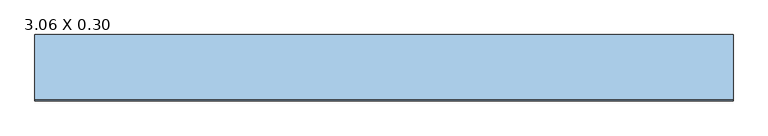
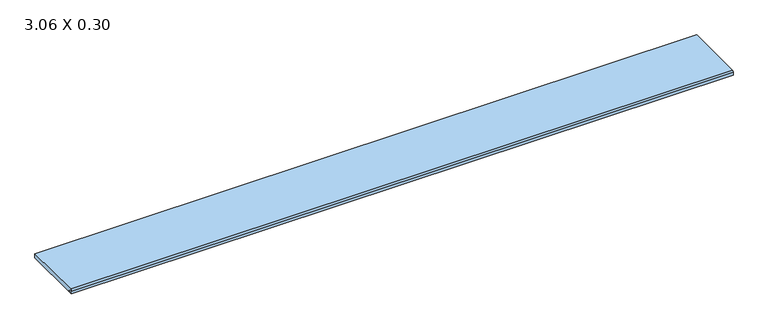
"""IFC4 building model written with IfcOpenShell, lengths in millimetres: window geometry, .CC_ND 300_PEDRA_PEITORIL RETO : 3.06 X 0.30."""

import ifcopenshell
import ifcopenshell.guid

model = None  # the IFC model being written
_history = None  # IfcOwnerHistory: only IFC2X3 demands one
_inside = {}  # id of a spatial element -> (the spatial element, [elements in it])
_under = {}  # id of a project, library or spatial element -> (it, [spatial elements below it])
_declared = {}  # id of a project -> (the project, [libraries it declares])
_typed = {}  # id of a type object -> (the type object, [elements of that type])
_made_of = {}  # id of a material, layer set ... -> (it, [elements and type objects made of it])


def new_model(schema):
    """Start an empty IFC model of exactly this schema.

    Asked for "IFC4X3", IfcOpenShell would pick the latest addendum, in which some entities
    have other attributes; the version numbers below select the first issue.
    IFC2X3 requires an IfcOwnerHistory on every rooted entity: one is made here for all.
    """
    global model, _history
    if schema == "IFC4X3":
        model = ifcopenshell.file(schema_version=(4, 3, 0, 0))
    else:
        model = ifcopenshell.file(schema=schema)
    _inside.clear()
    _under.clear()
    _declared.clear()
    _typed.clear()
    _made_of.clear()
    _history = None
    if model.schema == "IFC2X3":
        org = make("IfcOrganization", Name="unknown")
        user = make(
            "IfcPersonAndOrganization",
            ThePerson=make("IfcPerson", FamilyName="unknown"),
            TheOrganization=org,
        )
        app = make(
            "IfcApplication",
            ApplicationDeveloper=org,
            Version="unknown",
            ApplicationFullName="unknown",
            ApplicationIdentifier="unknown",
        )
        _history = make(
            "IfcOwnerHistory",
            OwningUser=user,
            OwningApplication=app,
            ChangeAction="ADDED",
            CreationDate=0,
        )
    return model


def make(cls, **values):
    """One entity of the class cls with the attributes given. An attribute that is None is left unset."""
    return model.create_entity(
        cls, **{name: value for name, value in values.items() if value is not None}
    )


def rooted(cls, **values):
    """An entity with a GlobalId (a new one), such as an element, a storey or a relation."""
    return make(cls, GlobalId=ifcopenshell.guid.new(), OwnerHistory=_history, **values)


def si_unit(unit_type, name, prefix=None):
    """IfcSIUnit, for example si_unit("LENGTHUNIT", "METRE", prefix="MILLI")."""
    return make("IfcSIUnit", UnitType=unit_type, Prefix=prefix, Name=name)


def assignment(units):
    """IfcUnitAssignment: the units of a project."""
    return None if units is None else make("IfcUnitAssignment", Units=units)


def point(xyz):
    """IfcCartesianPoint."""
    return None if xyz is None else make("IfcCartesianPoint", Coordinates=xyz)


def direction(xyz):
    """IfcDirection."""
    return None if xyz is None else make("IfcDirection", DirectionRatios=xyz)


def frame(location, z_axis=None, x_axis=None):
    """IfcAxis2Placement3D, a coordinate frame: its origin and axes. An axis left out is left unset."""
    return make(
        "IfcAxis2Placement3D",
        Location=point(location),
        Axis=direction(z_axis),
        RefDirection=direction(x_axis),
    )


def frame_2d(location, x_axis=None):
    """IfcAxis2Placement2D, a coordinate frame in the plane: its origin and x axis."""
    return make(
        "IfcAxis2Placement2D", Location=point(location), RefDirection=direction(x_axis)
    )


def origin():
    """The frame at (0, 0, 0) with its axes left unset."""
    return frame((0.0, 0.0, 0.0))


def place(relative_to, where):
    """IfcLocalPlacement: puts the frame where relative to a parent placement (None: the world)."""
    return make(
        "IfcLocalPlacement", PlacementRelTo=relative_to, RelativePlacement=where
    )


def context(
    kind, dimensions, precision=None, world=None, true_north=None, identifier=None
):
    """IfcGeometricRepresentationContext, for example the 3D "Model" context."""
    return make(
        "IfcGeometricRepresentationContext",
        ContextIdentifier=identifier,
        ContextType=kind,
        CoordinateSpaceDimension=dimensions,
        Precision=precision,
        WorldCoordinateSystem=world,
        TrueNorth=true_north,
    )


def project(units=None, contexts=None):
    """IfcProject with its units and contexts."""
    return rooted(
        "IfcProject",
        Name="project",
        RepresentationContexts=contexts,
        UnitsInContext=assignment(units),
    )


def spatial(cls, under=None, at=None, **own):
    """A site, building, storey or space (cls), placed at a placement, below another one or the project."""
    s = rooted(cls, ObjectPlacement=at, **own)
    if under is not None:
        _under.setdefault(under.id(), (under, []))[1].append(s)
    return s


def polyline(points):
    """IfcPolyline through the points."""
    return make("IfcPolyline", Points=[point(p) for p in points])


def circle_curve(where, radius):
    """IfcCircle in the frame where."""
    return make("IfcCircle", Position=where, Radius=radius)


def trimmed(basis, trim1, trim2, sense, master):
    """IfcTrimmedCurve: the piece of a basis curve between two trims."""
    return make(
        "IfcTrimmedCurve",
        BasisCurve=basis,
        Trim1=trim1,
        Trim2=trim2,
        SenseAgreement=sense,
        MasterRepresentation=master,
    )


def segment(curve, same_sense, transition):
    """IfcCompositeCurveSegment."""
    return make(
        "IfcCompositeCurveSegment",
        Transition=transition,
        SameSense=same_sense,
        ParentCurve=curve,
    )


def composite_curve(segments, self_intersect=None):
    """IfcCompositeCurve: segments joined end to end."""
    return make("IfcCompositeCurve", Segments=segments, SelfIntersect=self_intersect)


def outline(outer, holes=None, kind="AREA"):
    """IfcArbitraryClosedProfileDef: a profile drawn as a closed curve; with holes, ...WithVoids."""
    if holes is None:
        return make("IfcArbitraryClosedProfileDef", ProfileType=kind, OuterCurve=outer)
    return make(
        "IfcArbitraryProfileDefWithVoids",
        ProfileType=kind,
        OuterCurve=outer,
        InnerCurves=holes,
    )


def extrude(swept, where, along, depth):
    """IfcExtrudedAreaSolid: the profile swept, set in the frame where, extruded along a direction by depth."""
    return make(
        "IfcExtrudedAreaSolid",
        SweptArea=swept,
        Position=where,
        ExtrudedDirection=direction(along),
        Depth=depth,
    )


def shape(context_of_items, identifier, shape_type, items):
    """IfcShapeRepresentation: the items that make up one representation, for example the "Body"."""
    return make(
        "IfcShapeRepresentation",
        ContextOfItems=context_of_items,
        RepresentationIdentifier=identifier,
        RepresentationType=shape_type,
        Items=items,
    )


def source(mapping_origin, context_of_items, identifier, shape_type, items):
    """IfcRepresentationMap: a shape defined once, which mapped items show again and again."""
    return make(
        "IfcRepresentationMap",
        MappingOrigin=mapping_origin,
        MappedRepresentation=shape(context_of_items, identifier, shape_type, items),
    )


def transform(
    local_origin,
    x_axis=None,
    y_axis=None,
    z_axis=None,
    scale=None,
    scale2=None,
    scale3=None,
    uniform=True,
):
    """IfcCartesianTransformationOperator3D, or its non-uniform kind. x_axis, y_axis, z_axis: its Axis1, 2, 3."""
    if uniform:
        return make(
            "IfcCartesianTransformationOperator3D",
            Axis1=direction(x_axis),
            Axis2=direction(y_axis),
            LocalOrigin=point(local_origin),
            Scale=scale,
            Axis3=direction(z_axis),
        )
    return make(
        "IfcCartesianTransformationOperator3DnonUniform",
        Axis1=direction(x_axis),
        Axis2=direction(y_axis),
        LocalOrigin=point(local_origin),
        Scale=scale,
        Axis3=direction(z_axis),
        Scale2=scale2,
        Scale3=scale3,
    )


def mapped(mapping_source, mapping_target):
    """IfcMappedItem: shows the shape of a source again, moved by a transform."""
    return make(
        "IfcMappedItem", MappingSource=mapping_source, MappingTarget=mapping_target
    )


def made_of(thing, what):
    """Note that an element or type object is made of a material, layer set ...; save() writes the relation."""
    if what is not None:
        _made_of.setdefault(what.id(), (what, []))[1].append(thing)
    return thing


def element(
    cls,
    number,
    at=None,
    inside=None,
    cuts=None,
    type_object=None,
    material=None,
    context=None,
    identifier="Body",
    shape_type=None,
    held_by="IfcProductDefinitionShape",
    body=None,
    shapes=None,
    **own,
):
    """One element of the class cls, such as IfcWall. Its Tag is "e" and its number.

    at: its placement. inside: the storey or other place that contains it. cuts: it is an
    opening in that element (IfcRelVoidsElement). A single representation is given by context,
    identifier, shape_type and body (its items); several are given by shapes. held_by: the class
    of the entity that holds the representations. save() writes the other relations.
    """
    e = rooted(cls, Tag="e%d" % number, ObjectPlacement=at, **own)
    if body is not None:
        shapes = [shape(context, identifier, shape_type, body)]
    if shapes is not None:
        e.Representation = make(held_by, Representations=shapes)
    if inside is not None:
        _inside.setdefault(inside.id(), (inside, []))[1].append(e)
    if cuts is not None:
        rooted(
            "IfcRelVoidsElement", RelatingBuildingElement=cuts, RelatedOpeningElement=e
        )
    if type_object is not None:
        _typed.setdefault(type_object.id(), (type_object, []))[1].append(e)
    return made_of(e, material)


def aggregate(whole, parts):
    """IfcRelAggregates: a whole, such as a stair, and the parts it consists of."""
    return rooted("IfcRelAggregates", RelatingObject=whole, RelatedObjects=parts)


def save(model, path):
    """Write the relations noted so far, then the file.

    IfcRelAggregates (storeys below a building ...), IfcRelContainedInSpatialStructure (elements
    in a storey), IfcRelDefinesByType, IfcRelAssociatesMaterial and IfcRelDeclares: one each for
    every whole, place, type object, material and project.
    """
    for whole, parts in _under.values():
        aggregate(whole, parts)
    for where, things in _inside.values():
        rooted(
            "IfcRelContainedInSpatialStructure",
            RelatedElements=things,
            RelatingStructure=where,
        )
    for kind, things in _typed.values():
        rooted("IfcRelDefinesByType", RelatedObjects=things, RelatingType=kind)
    for what, things in _made_of.values():
        rooted("IfcRelAssociatesMaterial", RelatedObjects=things, RelatingMaterial=what)
    for by, libraries in _declared.values():
        rooted("IfcRelDeclares", RelatingContext=by, RelatedDefinitions=libraries)
    model.write(path)


def window_3_06_x_0_30_1a8a3462(model_context):
    return source(origin(), model_context, "Body", "SweptSolid", [
        extrude(outline(composite_curve([segment(polyline([(-132.5083081, 1480.0), (-132.5083081, 1488.1993124), (-137.2619526, 1488.1993124), (-137.2619526, 1480.0), (-148.0, 1480.0), (-148.0, 1493.3808343)]), True, "CONTINUOUS"), segment(trimmed(circle_curve(frame_2d((-141.3808343, 1493.3808343)), 6.6191657), [point((-148.0, 1493.3808343))], [point((-141.3808343, 1500.0))], False, "CARTESIAN"), True, "CONTINUOUS"), segment(polyline([(-141.3808343, 1500.0), (143.7, 1500.0), (143.7, 1480.0), (-132.5083081, 1480.0)]), True, "CONTINUOUS")], self_intersect=False)), frame((-1530.0, 0.0, 0.0), z_axis=(1.0, 0.0, 0.0), x_axis=(0.0, 1.0, 0.0)), (0.0, 0.0, 1.0), 3060.0),
    ])


if __name__ == "__main__":
    model = new_model("IFC4")
    model_context = context("Model", 3, world=origin())
    ifc_project = project(units=[si_unit("LENGTHUNIT", "METRE", prefix="MILLI")], contexts=[model_context])
    site = spatial("IfcSite", under=ifc_project)
    building = spatial("IfcBuilding", under=site)
    placement = place(None, origin())
    window_3_06_x_0_30_shape = window_3_06_x_0_30_1a8a3462(model_context)
    element("IfcWindow", 1, ObjectType=".CC_ND 300_PEDRA_PEITORIL RETO : 3.06 X 0.30", at=placement, inside=building, context=model_context, shape_type="MappedRepresentation", body=[
        mapped(window_3_06_x_0_30_shape, transform((0.0, 0.0, 0.0), x_axis=(1.0, 0.0, 0.0), y_axis=(0.0, 1.0, 0.0), z_axis=(0.0, 0.0, 1.0))),
    ])
    save(model, "model.ifc")

# Revit data of these elements
# Type ".CC_ND 300_PEDRA_PEITORIL RETO : 3.06 X 0.30"
#   Type Mark = "70"
#   Largura da pedra [instance default] = 0.26 m
#   Extensão interior peitoril [instance default] = 0.03 m
#   Extensão exterior peitoril [instance default] = 0.03 m
#   Espessura = 0.02 m
#   Comprimento = 3.06 m
#   Altura-padrão do peitoril = 1.48 m
#   Peitoril = .GRANITO_BRANCO_ITAUNAS
#   Rough Width = 0
#   Rough Height = 0
#   Height = 0
#   Wall Closure = (empty or 0)
#   Width = 0
# Element 1 (IfcWindow, ".CC_ND 300_PEDRA_PEITORIL RETO : 3.06 X 0.30")
#   Largura da pedra = 0.2917 m
#   Extensão interior peitoril = 0.0257 m
#   Materials on its faces: ".GRANITO_BRANCO_ITAUNAS"
# Materials
#   ".GRANITO_BRANCO_ITAUNAS": class ".CC_PEDRA REVEST.", colour RGB 202 195 174, transparency 0, Description = "Revestimento em granito", Cost = 0
